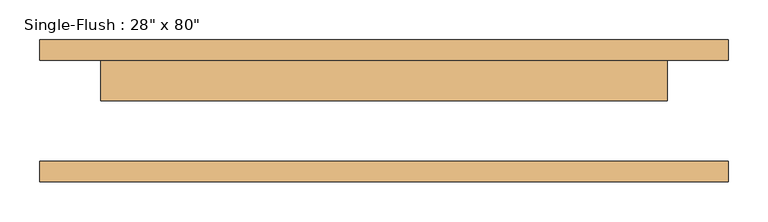
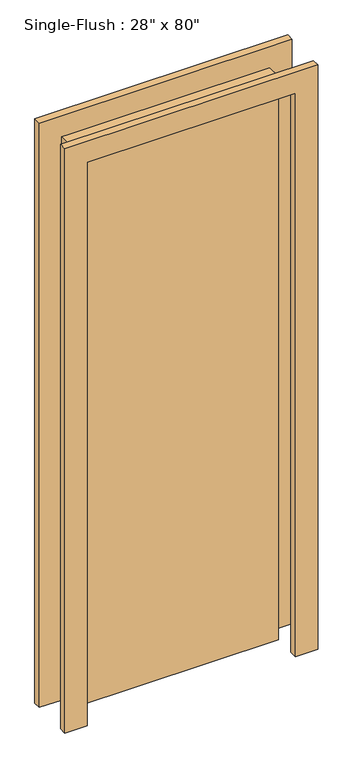
"""IFC4 building model written with IfcOpenShell, lengths in millimetres: door geometry."""

import ifcopenshell
import ifcopenshell.guid

model = None  # the IFC model being written
_history = None  # IfcOwnerHistory: only IFC2X3 demands one
_inside = {}  # id of a spatial element -> (the spatial element, [elements in it])
_under = {}  # id of a project, library or spatial element -> (it, [spatial elements below it])
_declared = {}  # id of a project -> (the project, [libraries it declares])
_typed = {}  # id of a type object -> (the type object, [elements of that type])
_made_of = {}  # id of a material, layer set ... -> (it, [elements and type objects made of it])


def new_model(schema):
    """Start an empty IFC model of exactly this schema.

    Asked for "IFC4X3", IfcOpenShell would pick the latest addendum, in which some entities
    have other attributes; the version numbers below select the first issue.
    IFC2X3 requires an IfcOwnerHistory on every rooted entity: one is made here for all.
    """
    global model, _history
    if schema == "IFC4X3":
        model = ifcopenshell.file(schema_version=(4, 3, 0, 0))
    else:
        model = ifcopenshell.file(schema=schema)
    _inside.clear()
    _under.clear()
    _declared.clear()
    _typed.clear()
    _made_of.clear()
    _history = None
    if model.schema == "IFC2X3":
        org = make("IfcOrganization", Name="unknown")
        user = make(
            "IfcPersonAndOrganization",
            ThePerson=make("IfcPerson", FamilyName="unknown"),
            TheOrganization=org,
        )
        app = make(
            "IfcApplication",
            ApplicationDeveloper=org,
            Version="unknown",
            ApplicationFullName="unknown",
            ApplicationIdentifier="unknown",
        )
        _history = make(
            "IfcOwnerHistory",
            OwningUser=user,
            OwningApplication=app,
            ChangeAction="ADDED",
            CreationDate=0,
        )
    return model


def make(cls, **values):
    """One entity of the class cls with the attributes given. An attribute that is None is left unset."""
    return model.create_entity(
        cls, **{name: value for name, value in values.items() if value is not None}
    )


def rooted(cls, **values):
    """An entity with a GlobalId (a new one), such as an element, a storey or a relation."""
    return make(cls, GlobalId=ifcopenshell.guid.new(), OwnerHistory=_history, **values)


def si_unit(unit_type, name, prefix=None):
    """IfcSIUnit, for example si_unit("LENGTHUNIT", "METRE", prefix="MILLI")."""
    return make("IfcSIUnit", UnitType=unit_type, Prefix=prefix, Name=name)


def assignment(units):
    """IfcUnitAssignment: the units of a project."""
    return None if units is None else make("IfcUnitAssignment", Units=units)


def point(xyz):
    """IfcCartesianPoint."""
    return None if xyz is None else make("IfcCartesianPoint", Coordinates=xyz)


def direction(xyz):
    """IfcDirection."""
    return None if xyz is None else make("IfcDirection", DirectionRatios=xyz)


def frame(location, z_axis=None, x_axis=None):
    """IfcAxis2Placement3D, a coordinate frame: its origin and axes. An axis left out is left unset."""
    return make(
        "IfcAxis2Placement3D",
        Location=point(location),
        Axis=direction(z_axis),
        RefDirection=direction(x_axis),
    )


def origin():
    """The frame at (0, 0, 0) with its axes left unset."""
    return frame((0.0, 0.0, 0.0))


def origin_with_axes():
    """The frame at (0, 0, 0) with the z axis (0, 0, 1) and the x axis (1, 0, 0) written out."""
    return frame((0.0, 0.0, 0.0), z_axis=(0.0, 0.0, 1.0), x_axis=(1.0, 0.0, 0.0))


def place(relative_to, where):
    """IfcLocalPlacement: puts the frame where relative to a parent placement (None: the world)."""
    return make(
        "IfcLocalPlacement", PlacementRelTo=relative_to, RelativePlacement=where
    )


def context(
    kind, dimensions, precision=None, world=None, true_north=None, identifier=None
):
    """IfcGeometricRepresentationContext, for example the 3D "Model" context."""
    return make(
        "IfcGeometricRepresentationContext",
        ContextIdentifier=identifier,
        ContextType=kind,
        CoordinateSpaceDimension=dimensions,
        Precision=precision,
        WorldCoordinateSystem=world,
        TrueNorth=true_north,
    )


def project(units=None, contexts=None):
    """IfcProject with its units and contexts."""
    return rooted(
        "IfcProject",
        Name="project",
        RepresentationContexts=contexts,
        UnitsInContext=assignment(units),
    )


def spatial(cls, under=None, at=None, **own):
    """A site, building, storey or space (cls), placed at a placement, below another one or the project."""
    s = rooted(cls, ObjectPlacement=at, **own)
    if under is not None:
        _under.setdefault(under.id(), (under, []))[1].append(s)
    return s


def polyline(points):
    """IfcPolyline through the points."""
    return make("IfcPolyline", Points=[point(p) for p in points])


def outline(outer, holes=None, kind="AREA"):
    """IfcArbitraryClosedProfileDef: a profile drawn as a closed curve; with holes, ...WithVoids."""
    if holes is None:
        return make("IfcArbitraryClosedProfileDef", ProfileType=kind, OuterCurve=outer)
    return make(
        "IfcArbitraryProfileDefWithVoids",
        ProfileType=kind,
        OuterCurve=outer,
        InnerCurves=holes,
    )


def extrude(swept, where, along, depth):
    """IfcExtrudedAreaSolid: the profile swept, set in the frame where, extruded along a direction by depth."""
    return make(
        "IfcExtrudedAreaSolid",
        SweptArea=swept,
        Position=where,
        ExtrudedDirection=direction(along),
        Depth=depth,
    )


def shape(context_of_items, identifier, shape_type, items):
    """IfcShapeRepresentation: the items that make up one representation, for example the "Body"."""
    return make(
        "IfcShapeRepresentation",
        ContextOfItems=context_of_items,
        RepresentationIdentifier=identifier,
        RepresentationType=shape_type,
        Items=items,
    )


def source(mapping_origin, context_of_items, identifier, shape_type, items):
    """IfcRepresentationMap: a shape defined once, which mapped items show again and again."""
    return make(
        "IfcRepresentationMap",
        MappingOrigin=mapping_origin,
        MappedRepresentation=shape(context_of_items, identifier, shape_type, items),
    )


def transform(
    local_origin,
    x_axis=None,
    y_axis=None,
    z_axis=None,
    scale=None,
    scale2=None,
    scale3=None,
    uniform=True,
):
    """IfcCartesianTransformationOperator3D, or its non-uniform kind. x_axis, y_axis, z_axis: its Axis1, 2, 3."""
    if uniform:
        return make(
            "IfcCartesianTransformationOperator3D",
            Axis1=direction(x_axis),
            Axis2=direction(y_axis),
            LocalOrigin=point(local_origin),
            Scale=scale,
            Axis3=direction(z_axis),
        )
    return make(
        "IfcCartesianTransformationOperator3DnonUniform",
        Axis1=direction(x_axis),
        Axis2=direction(y_axis),
        LocalOrigin=point(local_origin),
        Scale=scale,
        Axis3=direction(z_axis),
        Scale2=scale2,
        Scale3=scale3,
    )


def mapped(mapping_source, mapping_target):
    """IfcMappedItem: shows the shape of a source again, moved by a transform."""
    return make(
        "IfcMappedItem", MappingSource=mapping_source, MappingTarget=mapping_target
    )


def made_of(thing, what):
    """Note that an element or type object is made of a material, layer set ...; save() writes the relation."""
    if what is not None:
        _made_of.setdefault(what.id(), (what, []))[1].append(thing)
    return thing


def element(
    cls,
    number,
    at=None,
    inside=None,
    cuts=None,
    type_object=None,
    material=None,
    context=None,
    identifier="Body",
    shape_type=None,
    held_by="IfcProductDefinitionShape",
    body=None,
    shapes=None,
    **own,
):
    """One element of the class cls, such as IfcWall. Its Tag is "e" and its number.

    at: its placement. inside: the storey or other place that contains it. cuts: it is an
    opening in that element (IfcRelVoidsElement). A single representation is given by context,
    identifier, shape_type and body (its items); several are given by shapes. held_by: the class
    of the entity that holds the representations. save() writes the other relations.
    """
    e = rooted(cls, Tag="e%d" % number, ObjectPlacement=at, **own)
    if body is not None:
        shapes = [shape(context, identifier, shape_type, body)]
    if shapes is not None:
        e.Representation = make(held_by, Representations=shapes)
    if inside is not None:
        _inside.setdefault(inside.id(), (inside, []))[1].append(e)
    if cuts is not None:
        rooted(
            "IfcRelVoidsElement", RelatingBuildingElement=cuts, RelatedOpeningElement=e
        )
    if type_object is not None:
        _typed.setdefault(type_object.id(), (type_object, []))[1].append(e)
    return made_of(e, material)


def aggregate(whole, parts):
    """IfcRelAggregates: a whole, such as a stair, and the parts it consists of."""
    return rooted("IfcRelAggregates", RelatingObject=whole, RelatedObjects=parts)


def save(model, path):
    """Write the relations noted so far, then the file.

    IfcRelAggregates (storeys below a building ...), IfcRelContainedInSpatialStructure (elements
    in a storey), IfcRelDefinesByType, IfcRelAssociatesMaterial and IfcRelDeclares: one each for
    every whole, place, type object, material and project.
    """
    for whole, parts in _under.values():
        aggregate(whole, parts)
    for where, things in _inside.values():
        rooted(
            "IfcRelContainedInSpatialStructure",
            RelatedElements=things,
            RelatingStructure=where,
        )
    for kind, things in _typed.values():
        rooted("IfcRelDefinesByType", RelatedObjects=things, RelatingType=kind)
    for what, things in _made_of.values():
        rooted("IfcRelAssociatesMaterial", RelatedObjects=things, RelatingMaterial=what)
    for by, libraries in _declared.values():
        rooted("IfcRelDeclares", RelatingContext=by, RelatedDefinitions=libraries)
    model.write(path)


def door_7f94203e(model_context):
    return source(origin(), model_context, "Body", "SweptSolid", [
        extrude(outline(polyline([(2108.2, -431.8), (0.0, -431.8), (0.0, -355.6), (2032.0, -355.6), (2032.0, 355.6), (0.0, 355.6), (0.0, 431.8), (2108.2, 431.8), (2108.2, -431.8)])), frame((0.0, 63.5, 0.0), z_axis=(0.0, 1.0, 0.0), x_axis=(0.0, 0.0, 1.0)), (0.0, 0.0, 1.0), 25.4),
        extrude(outline(polyline([(2108.2, 431.8), (2108.2, -431.8), (0.0, -431.8), (0.0, -355.6), (2032.0, -355.6), (2032.0, 355.6), (0.0, 355.6), (0.0, 431.8), (2108.2, 431.8)])), frame((0.0, -88.9, 0.0), z_axis=(0.0, 1.0, 0.0), x_axis=(0.0, 0.0, 1.0)), (0.0, 0.0, 1.0), 25.4),
        extrude(outline(polyline([(355.6, 12.7), (-355.6, 12.7), (-355.6, 63.5), (355.6, 63.5), (355.6, 12.7)])), origin_with_axes(), (0.0, 0.0, 1.0), 2032.0),
    ])


if __name__ == "__main__":
    model = new_model("IFC4")
    model_context = context("Model", 3, world=origin())
    ifc_project = project(units=[si_unit("LENGTHUNIT", "METRE", prefix="MILLI")], contexts=[model_context])
    site = spatial("IfcSite", under=ifc_project)
    building = spatial("IfcBuilding", under=site)
    placement = place(None, origin())
    door_shape = door_7f94203e(model_context)
    element("IfcDoor", 1, ObjectType="Single-Flush : 28\" x 80\"", at=placement, inside=building, context=model_context, shape_type="MappedRepresentation", body=[
        mapped(door_shape, transform((0.0, 0.0, 0.0), x_axis=(1.0, 0.0, 0.0), y_axis=(0.0, 1.0, 0.0), z_axis=(0.0, 0.0, 1.0))),
    ])
    save(model, "model.ifc")

# Revit data of these elements
# Type "Single-Flush : 28\" x 80\""
#   Type Mark = "13"
#   Construction Type Id = "MDOOR"
#   Assembly Code = "C1020"
#   Analytic Construction = "Metal"
#   Thickness = 0' - 2"
#   Heat Transfer Coefficient (U) = 0.651978 BTU/(h·ft²·°F)
#   Height = 6' - 8"
#   Trim Projection Ext = 0' - 1"
#   Trim Projection Int = 0' - 1"
#   Trim Width = 0' - 3"
#   Width = 2' - 4"
#   Define Thermal Properties by = 1
#   Door Material = Door - Panel
#   Frame Material = Door - Frame
#   Visual Light Transmittance = 0
#   Solar Heat Gain Coefficient = 0
#   Function = (empty or 0)
#   Wall Closure = (empty or 0)
# Element 1 (IfcDoor, "Single-Flush : 28\" x 80\"")
#   Materials on its faces: "Door - Frame", "Door - Panel"
# Materials
#   "Door - Panel": class "Wood", colour RGB 210 159 95, transparency 0, Cost = 0
#   "Door - Frame": class "Miscellaneous", colour RGB 118 70 51, transparency 0, Cost = 0
